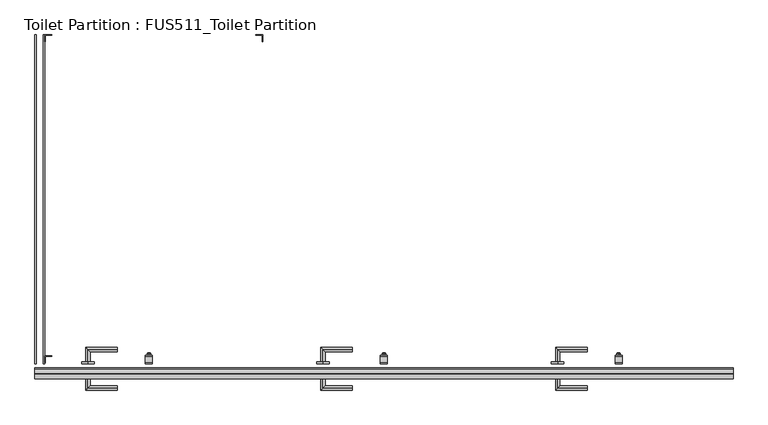
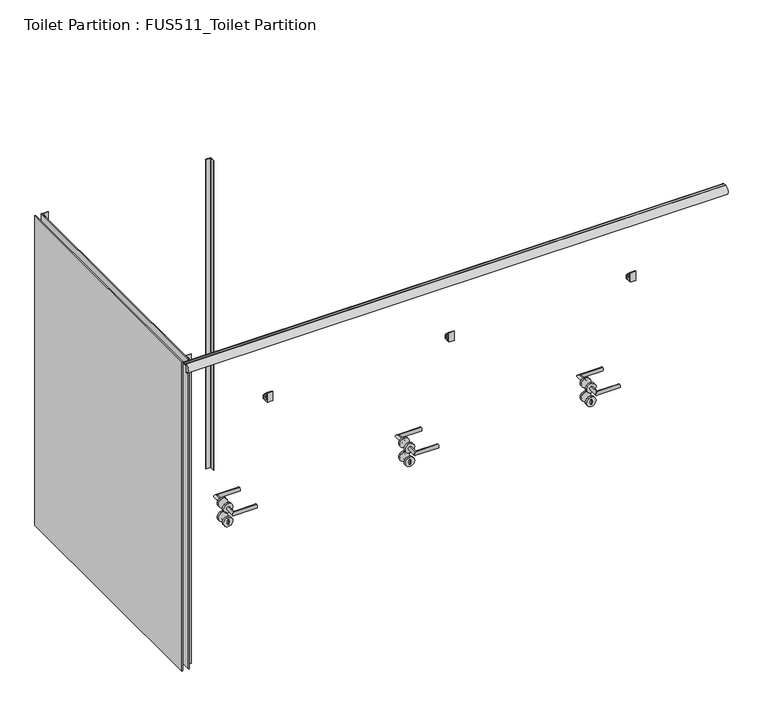
"""IFC4 building model written with IfcOpenShell, lengths in millimetres: furniture geometry, Toilet Partition : FUS511_Toilet Partition."""

from ifc_helpers import new_model, si_unit, point, frame, frame_2d, origin, place, context, project, spatial, polyline, circle_curve, ellipse_curve, trimmed, segment, composite_curve, outline, extrude, source, transform, mapped, element, save
from ifc_brep_helpers import plane_surface, cylinder_surface, revolved_surface, extruded_surface, advanced_brep


def toilet_partition_fus511_toilet_partition_80c0e7f6(model_context):
    return source(origin(), model_context, "Body", "SolidModel", [
        extrude(outline(composite_curve([segment(trimmed(circle_curve(frame_2d((-1451.3856706, 1892.2118377)), 1.0008364), [point((-1451.3856706, 1893.2126742))], [point((-1452.386507, 1892.2118377))], True, "CARTESIAN"), True, "CONTINUOUS"), segment(polyline([(-1452.386507, 1892.2118377), (-1452.386507, 1865.1892547), (-1453.3873434, 1865.1892547)]), True, "CONTINUOUS"), segment(trimmed(circle_curve(frame_2d((-1453.3873434, 1866.1900911)), 1.0008364), [point((-1453.3873434, 1865.1892547))], [point((-1454.3881798, 1866.1900911))], False, "CARTESIAN"), True, "CONTINUOUS"), segment(polyline([(-1454.3881798, 1866.1900911), (-1454.3881798, 1895.214347), (-1425.3639239, 1895.214347)]), True, "CONTINUOUS"), segment(trimmed(circle_curve(frame_2d((-1425.3639239, 1894.2135106)), 1.0008364), [point((-1425.3639239, 1895.214347))], [point((-1424.3630875, 1894.2135106))], False, "CARTESIAN"), True, "CONTINUOUS"), segment(polyline([(-1424.3630875, 1894.2135106), (-1424.3630875, 1893.2126742), (-1451.3856706, 1893.2126742)]), True, "CONTINUOUS")], self_intersect=False)), frame((0.0, 0.0, 100.0), z_axis=(0.0, 0.0, 1.0), x_axis=(1.0, 0.0, 0.0)), (0.0, 0.0, 1.0), 1800.0),
        extrude(outline(composite_curve([segment(trimmed(circle_curve(frame_2d((-1451.3856706, 527.0159753)), 1.0008364), [point((-1451.3856706, 528.0168117))], [point((-1452.386507, 527.0159753))], True, "CARTESIAN"), True, "CONTINUOUS"), segment(polyline([(-1452.386507, 527.0159753), (-1452.386507, 499.9933923), (-1453.3873434, 499.9933923)]), True, "CONTINUOUS"), segment(trimmed(circle_curve(frame_2d((-1453.3873434, 500.9942287)), 1.0008364), [point((-1453.3873434, 499.9933923))], [point((-1454.3881798, 500.9942287))], False, "CARTESIAN"), True, "CONTINUOUS"), segment(polyline([(-1454.3881798, 500.9942287), (-1454.3881798, 530.0184846), (-1425.3639239, 530.0184846)]), True, "CONTINUOUS"), segment(trimmed(circle_curve(frame_2d((-1425.3639239, 529.0176481)), 1.0008364), [point((-1425.3639239, 530.0184846))], [point((-1424.3630875, 529.0176481))], False, "CARTESIAN"), True, "CONTINUOUS"), segment(polyline([(-1424.3630875, 529.0176481), (-1424.3630875, 528.0168117), (-1451.3856706, 528.0168117)]), True, "CONTINUOUS")], self_intersect=False)), frame((0.0, 0.0, 100.0), z_axis=(0.0, 0.0, 1.0), x_axis=(1.0, 0.0, 0.0)), (0.0, 0.0, 1.0), 1800.0),
        extrude(outline(polyline([(-1454.3881798, 495.214347), (-1459.3881798, 495.214347), (-1459.3881798, 1895.214347), (-1454.3881798, 1895.214347), (-1454.3881798, 495.214347)])), frame((0.0, 0.0, 100.0), z_axis=(0.0, 0.0, 1.0), x_axis=(1.0, 0.0, 0.0)), (0.0, 0.0, 1.0), 1800.0),
        extrude(outline(polyline([(-1490.3881798, 495.214347), (-1495.3881798, 495.214347), (-1495.3881798, 1895.214347), (-1490.3881798, 1895.214347), (-1490.3881798, 495.214347)])), frame((0.0, 0.0, 100.0), z_axis=(0.0, 0.0, 1.0), x_axis=(1.0, 0.0, 0.0)), (0.0, 0.0, 1.0), 1800.0),
        advanced_brep(
        [(726.3556515, 505.214347, 893.5), (726.3556515, 505.214347, 946.5), (726.3556515, 505.214347, 934.6347495), (726.3556515, 505.214347, 904.6347495), (726.3556515, 495.214347, 893.5), (726.3556515, 495.214347, 946.5), (726.3556515, 499.9019579, 904.6347495), (726.3556515, 499.9019579, 934.6347495)],
        [
            (0, 1, circle_curve(frame((726.3556515, 505.214347, 920.0), z_axis=(0.0, 1.0, 0.0), x_axis=(0.0, 0.0, 1.0)), 26.5)),
            (1, 0, circle_curve(frame((726.3556515, 505.214347, 920.0), z_axis=(0.0, 1.0, 0.0), x_axis=(0.0, 0.0, 1.0)), 26.5)),
            (2, 3, ellipse_curve(frame((726.3556515, 505.214347, 919.6347495), z_axis=(0.0, -1.0, 0.0), x_axis=(0.0, 0.0, 1.0)), 15.0, 5.0)),
            (3, 2, ellipse_curve(frame((726.3556515, 505.214347, 919.6347495), z_axis=(0.0, -1.0, 0.0), x_axis=(0.0, 0.0, 1.0)), 15.0, 5.0)),
            (4, 5, circle_curve(frame((726.3556515, 495.214347, 920.0), z_axis=(0.0, -1.0, 0.0), x_axis=(0.0, 0.0, 1.0)), 26.5)),
            (5, 4, circle_curve(frame((726.3556515, 495.214347, 920.0), z_axis=(0.0, -1.0, 0.0), x_axis=(0.0, 0.0, 1.0)), 26.5)),
            (0, 4),
            (5, 1),
            (6, 7, ellipse_curve(frame((726.3556515, 499.9019579, 919.6347495), z_axis=(0.0, 1.0, 0.0), x_axis=(0.0, 0.0, 1.0)), 15.0, 5.0)),
            (7, 6, ellipse_curve(frame((726.3556515, 499.9019579, 919.6347495), z_axis=(0.0, 1.0, 0.0), x_axis=(0.0, 0.0, 1.0)), 15.0, 5.0)),
            (6, 3),
            (2, 7),
        ],
        [
            plane_surface(frame((726.3556515, 505.214347, 946.5), z_axis=(0.0, 1.0, 0.0), x_axis=(1.0, 0.0, 0.0))),
            plane_surface(frame((726.3556515, 495.214347, 946.5), z_axis=(0.0, -1.0, 0.0), x_axis=(-1.0, 0.0, 0.0))),
            cylinder_surface(frame((726.3556515, 495.214347, 920.0), z_axis=(0.0, 1.0, 0.0), x_axis=(0.0, 0.0, 1.0)), 26.5),
            plane_surface(frame((726.3556515, 499.9019579, 934.6347495), z_axis=(0.0, 1.0, 0.0), x_axis=(-1.0, 0.0, 0.0))),
            extruded_surface(trimmed(ellipse_curve(frame((726.3556515, 499.9019579, 919.6347495), z_axis=(0.0, 1.0, 0.0), x_axis=(0.0, 0.0, 1.0)), 15.0, 5.0), [point((726.3556515, 499.9019579, 904.6347495))], [point((726.3556515, 499.9019579, 934.6347495))], True, "CARTESIAN"), (0.0, -5.312388999999996, 0.0), 5.312388999999996),
            extruded_surface(trimmed(ellipse_curve(frame((726.3556515, 499.9019579, 919.6347495), z_axis=(0.0, 1.0, 0.0), x_axis=(0.0, 0.0, 1.0)), 15.0, 5.0), [point((726.3556515, 499.9019579, 934.6347495))], [point((726.3556515, 499.9019579, 904.6347495))], True, "CARTESIAN"), (0.0, -5.312388999999996, 0.0), 5.312388999999996),
        ],
        [
            (0, [[1, 2], [3, 4]]),
            (1, [[5, 6]]),
            (2, [[-1, 7, -6, 8]]),
            (2, [[-2, -8, -5, -7]]),
            (3, [[9, 10]]),
            (4, [[-9, 11, -3, 12]]),
            (5, [[-10, -12, -4, -11]]),
        ],
    ),
        advanced_brep(
        [(726.3556515, 505.214347, 990.5), (726.3556515, 505.214347, 1009.5), (726.3556515, 555.714347, 990.5), (726.3556515, 555.714347, 1009.5), (851.8556515, 555.714347, 990.5), (851.8556515, 555.714347, 1009.5)],
        [
            (0, 1, circle_curve(frame((726.3556515, 505.214347, 1000.0), z_axis=(0.0, -1.0, 0.0), x_axis=(0.0, 0.0, 1.0)), 9.5)),
            (1, 0, circle_curve(frame((726.3556515, 505.214347, 1000.0), z_axis=(0.0, -1.0, 0.0), x_axis=(0.0, 0.0, 1.0)), 9.5)),
            (0, 2),
            (2, 3, ellipse_curve(frame((726.3556515, 555.714347, 1000.0), z_axis=(-0.7071067811865486, -0.7071067811865465, 0.0), x_axis=(0.7071067811865465, -0.7071067811865485, 0.0)), 13.4350288, 9.5)),
            (3, 1),
            (3, 2, ellipse_curve(frame((726.3556515, 555.714347, 1000.0), z_axis=(-0.7071067811865486, -0.7071067811865465, 0.0), x_axis=(0.7071067811865465, -0.7071067811865485, 0.0)), 13.4350288, 9.5)),
            (4, 5, circle_curve(frame((851.8556515, 555.714347, 1000.0), z_axis=(1.0, 0.0, 0.0), x_axis=(0.0, 0.0, 1.0)), 9.5)),
            (5, 4, circle_curve(frame((851.8556515, 555.714347, 1000.0), z_axis=(1.0, 0.0, 0.0), x_axis=(0.0, 0.0, 1.0)), 9.5)),
            (2, 4),
            (5, 3),
        ],
        [
            plane_surface(frame((716.8556515, 505.214347, 1000.0), z_axis=(0.0, -1.0, 0.0), x_axis=(0.0, 0.0, 1.0))),
            cylinder_surface(frame((726.3556515, 505.214347, 1000.0), z_axis=(0.0, -1.0, 0.0), x_axis=(0.0, 0.0, 1.0)), 9.5),
            plane_surface(frame((851.8556515, 565.214347, 1000.0), z_axis=(1.0, 0.0, 0.0), x_axis=(0.0, 0.0, 1.0))),
            cylinder_surface(frame((716.8556515, 555.714347, 1000.0), z_axis=(-1.0, 0.0, 0.0), x_axis=(0.0, 0.0, 1.0)), 9.5),
        ],
        [
            (0, [[1, 2]]),
            (1, [[-1, 3, 4, 5]]),
            (1, [[-2, -5, 6, -3]]),
            (2, [[7, 8]]),
            (3, [[-4, 9, -8, 10]]),
            (3, [[-6, -10, -7, -9]]),
        ],
    ),
        extrude(outline(composite_curve([segment(trimmed(circle_curve(frame_2d((1000.0, 726.3556515)), 26.5), [point((973.5, 726.3556515))], [point((1026.5, 726.3556515))], False, "CARTESIAN"), True, "CONTINUOUS"), segment(trimmed(circle_curve(frame_2d((1000.0, 726.3556515)), 26.5), [point((1026.5, 726.3556515))], [point((973.5, 726.3556515))], False, "CARTESIAN"), True, "CONTINUOUS")], self_intersect=False)), frame((0.0, 495.214347, 0.0), z_axis=(0.0, 1.0, 0.0), x_axis=(0.0, 0.0, 1.0)), (0.0, 0.0, 1.0), 10.0),
        advanced_brep(
        [(-271.279512, 505.214347, 893.5), (-271.279512, 505.214347, 946.5), (-271.279512, 505.214347, 934.6347495), (-271.279512, 505.214347, 904.6347495), (-271.279512, 495.214347, 893.5), (-271.279512, 495.214347, 946.5), (-271.279512, 499.9019579, 904.6347495), (-271.279512, 499.9019579, 934.6347495)],
        [
            (0, 1, circle_curve(frame((-271.279512, 505.214347, 920.0), z_axis=(0.0, 1.0, 0.0), x_axis=(0.0, 0.0, 1.0)), 26.5)),
            (1, 0, circle_curve(frame((-271.279512, 505.214347, 920.0), z_axis=(0.0, 1.0, 0.0), x_axis=(0.0, 0.0, 1.0)), 26.5)),
            (2, 3, ellipse_curve(frame((-271.279512, 505.214347, 919.6347495), z_axis=(0.0, -1.0, 0.0), x_axis=(0.0, 0.0, 1.0)), 15.0, 5.0)),
            (3, 2, ellipse_curve(frame((-271.279512, 505.214347, 919.6347495), z_axis=(0.0, -1.0, 0.0), x_axis=(0.0, 0.0, 1.0)), 15.0, 5.0)),
            (4, 5, circle_curve(frame((-271.279512, 495.214347, 920.0), z_axis=(0.0, -1.0, 0.0), x_axis=(0.0, 0.0, 1.0)), 26.5)),
            (5, 4, circle_curve(frame((-271.279512, 495.214347, 920.0), z_axis=(0.0, -1.0, 0.0), x_axis=(0.0, 0.0, 1.0)), 26.5)),
            (0, 4),
            (5, 1),
            (6, 7, ellipse_curve(frame((-271.279512, 499.9019579, 919.6347495), z_axis=(0.0, 1.0, 0.0), x_axis=(0.0, 0.0, 1.0)), 15.0, 5.0)),
            (7, 6, ellipse_curve(frame((-271.279512, 499.9019579, 919.6347495), z_axis=(0.0, 1.0, 0.0), x_axis=(0.0, 0.0, 1.0)), 15.0, 5.0)),
            (6, 3),
            (2, 7),
        ],
        [
            plane_surface(frame((-271.279512, 505.214347, 946.5), z_axis=(0.0, 1.0, 0.0), x_axis=(1.0, 0.0, 0.0))),
            plane_surface(frame((-271.279512, 495.214347, 946.5), z_axis=(0.0, -1.0, 0.0), x_axis=(-1.0, 0.0, 0.0))),
            cylinder_surface(frame((-271.279512, 495.214347, 920.0), z_axis=(0.0, 1.0, 0.0), x_axis=(0.0, 0.0, 1.0)), 26.5),
            plane_surface(frame((-271.279512, 499.9019579, 934.6347495), z_axis=(0.0, 1.0, 0.0), x_axis=(-1.0, 0.0, 0.0))),
            extruded_surface(trimmed(ellipse_curve(frame((-271.279512, 499.9019579, 919.6347495), z_axis=(0.0, 1.0, 0.0), x_axis=(0.0, 0.0, 1.0)), 15.0, 5.0), [point((-271.279512, 499.9019579, 904.6347495))], [point((-271.279512, 499.9019579, 934.6347495))], True, "CARTESIAN"), (0.0, -5.312388999999996, 0.0), 5.312388999999996),
            extruded_surface(trimmed(ellipse_curve(frame((-271.279512, 499.9019579, 919.6347495), z_axis=(0.0, 1.0, 0.0), x_axis=(0.0, 0.0, 1.0)), 15.0, 5.0), [point((-271.279512, 499.9019579, 934.6347495))], [point((-271.279512, 499.9019579, 904.6347495))], True, "CARTESIAN"), (0.0, -5.312388999999996, 0.0), 5.312388999999996),
        ],
        [
            (0, [[1, 2], [3, 4]]),
            (1, [[5, 6]]),
            (2, [[-1, 7, -6, 8]]),
            (2, [[-2, -8, -5, -7]]),
            (3, [[9, 10]]),
            (4, [[-9, 11, -3, 12]]),
            (5, [[-10, -12, -4, -11]]),
        ],
    ),
        advanced_brep(
        [(-271.279512, 505.214347, 990.5), (-271.279512, 505.214347, 1009.5), (-271.279512, 555.714347, 990.5), (-271.279512, 555.714347, 1009.5), (-145.779512, 555.714347, 990.5), (-145.779512, 555.714347, 1009.5)],
        [
            (0, 1, circle_curve(frame((-271.279512, 505.214347, 1000.0), z_axis=(0.0, -1.0, 0.0), x_axis=(0.0, 0.0, 1.0)), 9.5)),
            (1, 0, circle_curve(frame((-271.279512, 505.214347, 1000.0), z_axis=(0.0, -1.0, 0.0), x_axis=(0.0, 0.0, 1.0)), 9.5)),
            (0, 2),
            (2, 3, ellipse_curve(frame((-271.279512, 555.714347, 1000.0), z_axis=(-0.7071067811865486, -0.7071067811865465, 0.0), x_axis=(0.7071067811865465, -0.7071067811865485, 0.0)), 13.4350288, 9.5)),
            (3, 1),
            (3, 2, ellipse_curve(frame((-271.279512, 555.714347, 1000.0), z_axis=(-0.7071067811865486, -0.7071067811865465, 0.0), x_axis=(0.7071067811865465, -0.7071067811865485, 0.0)), 13.4350288, 9.5)),
            (4, 5, circle_curve(frame((-145.779512, 555.714347, 1000.0), z_axis=(1.0, 0.0, 0.0), x_axis=(0.0, 0.0, 1.0)), 9.5)),
            (5, 4, circle_curve(frame((-145.779512, 555.714347, 1000.0), z_axis=(1.0, 0.0, 0.0), x_axis=(0.0, 0.0, 1.0)), 9.5)),
            (2, 4),
            (5, 3),
        ],
        [
            plane_surface(frame((-280.779512, 505.214347, 1000.0), z_axis=(0.0, -1.0, 0.0), x_axis=(0.0, 0.0, 1.0))),
            cylinder_surface(frame((-271.279512, 505.214347, 1000.0), z_axis=(0.0, -1.0, 0.0), x_axis=(0.0, 0.0, 1.0)), 9.5),
            plane_surface(frame((-145.779512, 565.214347, 1000.0), z_axis=(1.0, 0.0, 0.0), x_axis=(0.0, 0.0, 1.0))),
            cylinder_surface(frame((-280.779512, 555.714347, 1000.0), z_axis=(-1.0, 0.0, 0.0), x_axis=(0.0, 0.0, 1.0)), 9.5),
        ],
        [
            (0, [[1, 2]]),
            (1, [[-1, 3, 4, 5]]),
            (1, [[-2, -5, 6, -3]]),
            (2, [[7, 8]]),
            (3, [[-4, 9, -8, 10]]),
            (3, [[-6, -10, -7, -9]]),
        ],
    ),
        extrude(outline(composite_curve([segment(trimmed(circle_curve(frame_2d((1000.0, -271.279512)), 26.5), [point((973.5, -271.279512))], [point((1026.5, -271.279512))], False, "CARTESIAN"), True, "CONTINUOUS"), segment(trimmed(circle_curve(frame_2d((1000.0, -271.279512)), 26.5), [point((1026.5, -271.279512))], [point((973.5, -271.279512))], False, "CARTESIAN"), True, "CONTINUOUS")], self_intersect=False)), frame((0.0, 495.214347, 0.0), z_axis=(0.0, 1.0, 0.0), x_axis=(0.0, 0.0, 1.0)), (0.0, 0.0, 1.0), 10.0),
        advanced_brep(
        [(-1270.2108466, 505.214347, 893.5), (-1270.2108466, 505.214347, 946.5), (-1270.2108466, 505.214347, 934.6347495), (-1270.2108466, 505.214347, 904.6347495), (-1270.2108466, 495.214347, 893.5), (-1270.2108466, 495.214347, 946.5), (-1270.2108466, 499.9019579, 904.6347495), (-1270.2108466, 499.9019579, 934.6347495)],
        [
            (0, 1, circle_curve(frame((-1270.2108466, 505.214347, 920.0), z_axis=(0.0, 1.0, 0.0), x_axis=(0.0, 0.0, 1.0)), 26.5)),
            (1, 0, circle_curve(frame((-1270.2108466, 505.214347, 920.0), z_axis=(0.0, 1.0, 0.0), x_axis=(0.0, 0.0, 1.0)), 26.5)),
            (2, 3, ellipse_curve(frame((-1270.2108466, 505.214347, 919.6347495), z_axis=(0.0, -1.0, 0.0), x_axis=(0.0, 0.0, 1.0)), 15.0, 5.0)),
            (3, 2, ellipse_curve(frame((-1270.2108466, 505.214347, 919.6347495), z_axis=(0.0, -1.0, 0.0), x_axis=(0.0, 0.0, 1.0)), 15.0, 5.0)),
            (4, 5, circle_curve(frame((-1270.2108466, 495.214347, 920.0), z_axis=(0.0, -1.0, 0.0), x_axis=(0.0, 0.0, 1.0)), 26.5)),
            (5, 4, circle_curve(frame((-1270.2108466, 495.214347, 920.0), z_axis=(0.0, -1.0, 0.0), x_axis=(0.0, 0.0, 1.0)), 26.5)),
            (0, 4),
            (5, 1),
            (6, 7, ellipse_curve(frame((-1270.2108466, 499.9019579, 919.6347495), z_axis=(0.0, 1.0, 0.0), x_axis=(0.0, 0.0, 1.0)), 15.0, 5.0)),
            (7, 6, ellipse_curve(frame((-1270.2108466, 499.9019579, 919.6347495), z_axis=(0.0, 1.0, 0.0), x_axis=(0.0, 0.0, 1.0)), 15.0, 5.0)),
            (6, 3),
            (2, 7),
        ],
        [
            plane_surface(frame((-1270.2108466, 505.214347, 946.5), z_axis=(0.0, 1.0, 0.0), x_axis=(1.0, 0.0, 0.0))),
            plane_surface(frame((-1270.2108466, 495.214347, 946.5), z_axis=(0.0, -1.0, 0.0), x_axis=(-1.0, 0.0, 0.0))),
            cylinder_surface(frame((-1270.2108466, 495.214347, 920.0), z_axis=(0.0, 1.0, 0.0), x_axis=(0.0, 0.0, 1.0)), 26.5),
            plane_surface(frame((-1270.2108466, 499.9019579, 934.6347495), z_axis=(0.0, 1.0, 0.0), x_axis=(-1.0, 0.0, 0.0))),
            extruded_surface(trimmed(ellipse_curve(frame((-1270.2108466, 499.9019579, 919.6347495), z_axis=(0.0, 1.0, 0.0), x_axis=(0.0, 0.0, 1.0)), 15.0, 5.0), [point((-1270.2108466, 499.9019579, 904.6347495))], [point((-1270.2108466, 499.9019579, 934.6347495))], True, "CARTESIAN"), (0.0, -5.312388999999996, 0.0), 5.312388999999996),
            extruded_surface(trimmed(ellipse_curve(frame((-1270.2108466, 499.9019579, 919.6347495), z_axis=(0.0, 1.0, 0.0), x_axis=(0.0, 0.0, 1.0)), 15.0, 5.0), [point((-1270.2108466, 499.9019579, 934.6347495))], [point((-1270.2108466, 499.9019579, 904.6347495))], True, "CARTESIAN"), (0.0, -5.312388999999996, 0.0), 5.312388999999996),
        ],
        [
            (0, [[1, 2], [3, 4]]),
            (1, [[5, 6]]),
            (2, [[-1, 7, -6, 8]]),
            (2, [[-2, -8, -5, -7]]),
            (3, [[9, 10]]),
            (4, [[-9, 11, -3, 12]]),
            (5, [[-10, -12, -4, -11]]),
        ],
    ),
        advanced_brep(
        [(-1270.2108466, 505.214347, 990.5), (-1270.2108466, 505.214347, 1009.5), (-1270.2108466, 555.714347, 990.5), (-1270.2108466, 555.714347, 1009.5), (-1144.7108466, 555.714347, 990.5), (-1144.7108466, 555.714347, 1009.5)],
        [
            (0, 1, circle_curve(frame((-1270.2108466, 505.214347, 1000.0), z_axis=(0.0, -1.0, 0.0), x_axis=(0.0, 0.0, 1.0)), 9.5)),
            (1, 0, circle_curve(frame((-1270.2108466, 505.214347, 1000.0), z_axis=(0.0, -1.0, 0.0), x_axis=(0.0, 0.0, 1.0)), 9.5)),
            (0, 2),
            (2, 3, ellipse_curve(frame((-1270.2108466, 555.714347, 1000.0), z_axis=(-0.7071067811865486, -0.7071067811865465, 0.0), x_axis=(0.7071067811865465, -0.7071067811865485, 0.0)), 13.4350288, 9.5)),
            (3, 1),
            (3, 2, ellipse_curve(frame((-1270.2108466, 555.714347, 1000.0), z_axis=(-0.7071067811865486, -0.7071067811865465, 0.0), x_axis=(0.7071067811865465, -0.7071067811865485, 0.0)), 13.4350288, 9.5)),
            (4, 5, circle_curve(frame((-1144.7108466, 555.714347, 1000.0), z_axis=(1.0, 0.0, 0.0), x_axis=(0.0, 0.0, 1.0)), 9.5)),
            (5, 4, circle_curve(frame((-1144.7108466, 555.714347, 1000.0), z_axis=(1.0, 0.0, 0.0), x_axis=(0.0, 0.0, 1.0)), 9.5)),
            (2, 4),
            (5, 3),
        ],
        [
            plane_surface(frame((-1279.7108466, 505.214347, 1000.0), z_axis=(0.0, -1.0, 0.0), x_axis=(0.0, 0.0, 1.0))),
            cylinder_surface(frame((-1270.2108466, 505.214347, 1000.0), z_axis=(0.0, -1.0, 0.0), x_axis=(0.0, 0.0, 1.0)), 9.5),
            plane_surface(frame((-1144.7108466, 565.214347, 1000.0), z_axis=(1.0, 0.0, 0.0), x_axis=(0.0, 0.0, 1.0))),
            cylinder_surface(frame((-1279.7108466, 555.714347, 1000.0), z_axis=(-1.0, 0.0, 0.0), x_axis=(0.0, 0.0, 1.0)), 9.5),
        ],
        [
            (0, [[1, 2]]),
            (1, [[-1, 3, 4, 5]]),
            (1, [[-2, -5, 6, -3]]),
            (2, [[7, 8]]),
            (3, [[-4, 9, -8, 10]]),
            (3, [[-6, -10, -7, -9]]),
        ],
    ),
        extrude(outline(composite_curve([segment(trimmed(circle_curve(frame_2d((1000.0, -1270.2108466)), 26.5), [point((973.5, -1270.2108466))], [point((1026.5, -1270.2108466))], False, "CARTESIAN"), True, "CONTINUOUS"), segment(trimmed(circle_curve(frame_2d((1000.0, -1270.2108466)), 26.5), [point((1026.5, -1270.2108466))], [point((973.5, -1270.2108466))], False, "CARTESIAN"), True, "CONTINUOUS")], self_intersect=False)), frame((0.0, 495.214347, 0.0), z_axis=(0.0, 1.0, 0.0), x_axis=(0.0, 0.0, 1.0)), (0.0, 0.0, 1.0), 10.0),
        advanced_brep(
        [(726.3556515, 444.214347, 893.5), (726.3556515, 444.214347, 946.5), (726.3556515, 444.214347, 934.6347495), (726.3556515, 444.214347, 904.6347495), (726.3556515, 454.214347, 893.5), (726.3556515, 454.214347, 946.5), (726.3556515, 449.526736, 904.6347495), (726.3556515, 449.526736, 934.6347495)],
        [
            (0, 1, circle_curve(frame((726.3556515, 444.214347, 920.0), z_axis=(0.0, -1.0, 0.0), x_axis=(0.0, 0.0, 1.0)), 26.5)),
            (1, 0, circle_curve(frame((726.3556515, 444.214347, 920.0), z_axis=(0.0, -1.0, 0.0), x_axis=(0.0, 0.0, 1.0)), 26.5)),
            (2, 3, ellipse_curve(frame((726.3556515, 444.214347, 919.6347495), z_axis=(0.0, 1.0, 0.0), x_axis=(0.0, 0.0, 1.0)), 15.0, 5.0)),
            (3, 2, ellipse_curve(frame((726.3556515, 444.214347, 919.6347495), z_axis=(0.0, 1.0, 0.0), x_axis=(0.0, 0.0, 1.0)), 15.0, 5.0)),
            (4, 5, circle_curve(frame((726.3556515, 454.214347, 920.0), z_axis=(0.0, 1.0, 0.0), x_axis=(0.0, 0.0, 1.0)), 26.5)),
            (5, 4, circle_curve(frame((726.3556515, 454.214347, 920.0), z_axis=(0.0, 1.0, 0.0), x_axis=(0.0, 0.0, 1.0)), 26.5)),
            (1, 5),
            (4, 0),
            (6, 7, ellipse_curve(frame((726.3556515, 449.526736, 919.6347495), z_axis=(0.0, -1.0, 0.0), x_axis=(0.0, 0.0, 1.0)), 15.0, 5.0)),
            (7, 6, ellipse_curve(frame((726.3556515, 449.526736, 919.6347495), z_axis=(0.0, -1.0, 0.0), x_axis=(0.0, 0.0, 1.0)), 15.0, 5.0)),
            (7, 2),
            (3, 6),
        ],
        [
            plane_surface(frame((726.3556515, 444.214347, 946.5), z_axis=(0.0, -1.0, 0.0), x_axis=(1.0, 0.0, 0.0))),
            plane_surface(frame((726.3556515, 454.214347, 946.5), z_axis=(0.0, 1.0, 0.0), x_axis=(-1.0, 0.0, 0.0))),
            cylinder_surface(frame((726.3556515, 454.214347, 920.0), z_axis=(0.0, -1.0, 0.0), x_axis=(0.0, 0.0, 1.0)), 26.5),
            plane_surface(frame((726.3556515, 449.526736, 934.6347495), z_axis=(0.0, -1.0, 0.0), x_axis=(-1.0, 0.0, 0.0))),
            extruded_surface(trimmed(ellipse_curve(frame((726.3556515, 454.8391251, 919.6347495), z_axis=(0.0, 1.0, 0.0), x_axis=(0.0, 0.0, 1.0)), 15.0, 5.0), [point((726.3556515, 454.8391251, 904.6347495))], [point((726.3556515, 454.8391251, 934.6347495))], True, "CARTESIAN"), (0.0, -5.312389099999962, 0.0), 5.312389099999962),
            extruded_surface(trimmed(ellipse_curve(frame((726.3556515, 454.8391251, 919.6347495), z_axis=(0.0, 1.0, 0.0), x_axis=(0.0, 0.0, 1.0)), 15.0, 5.0), [point((726.3556515, 454.8391251, 934.6347495))], [point((726.3556515, 454.8391251, 904.6347495))], True, "CARTESIAN"), (0.0, -5.312389099999962, 0.0), 5.312389099999962),
        ],
        [
            (0, [[1, 2], [3, 4]]),
            (1, [[5, 6]]),
            (2, [[7, -5, 8, -2]]),
            (2, [[-8, -6, -7, -1]]),
            (3, [[9, 10]]),
            (4, [[11, -4, 12, -10]]),
            (5, [[-12, -3, -11, -9]]),
        ],
    ),
        advanced_brep(
        [(726.3556515, 444.214347, 990.5), (726.3556515, 444.214347, 1009.5), (726.3556515, 393.714347, 1009.5), (726.3556515, 393.714347, 990.5), (851.8556515, 393.714347, 990.5), (851.8556515, 393.714347, 1009.5)],
        [
            (0, 1, circle_curve(frame((726.3556515, 444.214347, 1000.0), z_axis=(0.0, 1.0, 0.0), x_axis=(0.0, 0.0, 1.0)), 9.5)),
            (1, 0, circle_curve(frame((726.3556515, 444.214347, 1000.0), z_axis=(0.0, 1.0, 0.0), x_axis=(0.0, 0.0, 1.0)), 9.5)),
            (1, 2),
            (2, 3, ellipse_curve(frame((726.3556515, 393.714347, 1000.0), z_axis=(-0.7071067811865486, 0.7071067811865465, 0.0), x_axis=(0.7071067811865465, 0.7071067811865485, 0.0)), 13.4350288, 9.5)),
            (3, 0),
            (3, 2, ellipse_curve(frame((726.3556515, 393.714347, 1000.0), z_axis=(-0.7071067811865486, 0.7071067811865465, 0.0), x_axis=(0.7071067811865465, 0.7071067811865485, 0.0)), 13.4350288, 9.5)),
            (4, 5, circle_curve(frame((851.8556515, 393.714347, 1000.0), z_axis=(1.0, 0.0, 0.0), x_axis=(0.0, 0.0, 1.0)), 9.5)),
            (5, 4, circle_curve(frame((851.8556515, 393.714347, 1000.0), z_axis=(1.0, 0.0, 0.0), x_axis=(0.0, 0.0, 1.0)), 9.5)),
            (2, 5),
            (4, 3),
        ],
        [
            plane_surface(frame((716.8556515, 444.214347, 1000.0), z_axis=(0.0, 1.0, 0.0), x_axis=(0.0, 0.0, 1.0))),
            cylinder_surface(frame((726.3556515, 444.214347, 1000.0), z_axis=(0.0, 1.0, 0.0), x_axis=(0.0, 0.0, 1.0)), 9.5),
            plane_surface(frame((851.8556515, 384.214347, 1000.0), z_axis=(1.0, 0.0, 0.0), x_axis=(0.0, 0.0, 1.0))),
            cylinder_surface(frame((716.8556515, 393.714347, 1000.0), z_axis=(-1.0, 0.0, 0.0), x_axis=(0.0, 0.0, 1.0)), 9.5),
        ],
        [
            (0, [[1, 2]]),
            (1, [[3, 4, 5, -2]]),
            (1, [[-5, 6, -3, -1]]),
            (2, [[7, 8]]),
            (3, [[9, -7, 10, -4]]),
            (3, [[-10, -8, -9, -6]]),
        ],
    ),
        extrude(outline(composite_curve([segment(trimmed(circle_curve(frame_2d((1000.0, 726.3556515)), 26.5), [point((973.5, 726.3556515))], [point((1026.5, 726.3556515))], False, "CARTESIAN"), True, "CONTINUOUS"), segment(trimmed(circle_curve(frame_2d((1000.0, 726.3556515)), 26.5), [point((1026.5, 726.3556515))], [point((973.5, 726.3556515))], False, "CARTESIAN"), True, "CONTINUOUS")], self_intersect=False)), frame((0.0, 444.214347, 0.0), z_axis=(0.0, 1.0, 0.0), x_axis=(0.0, 0.0, 1.0)), (0.0, 0.0, 1.0), 10.0),
        advanced_brep(
        [(-271.279512, 444.214347, 893.5), (-271.279512, 444.214347, 946.5), (-271.279512, 444.214347, 934.6347495), (-271.279512, 444.214347, 904.6347495), (-271.279512, 454.214347, 893.5), (-271.279512, 454.214347, 946.5), (-271.279512, 449.526736, 904.6347495), (-271.279512, 449.526736, 934.6347495)],
        [
            (0, 1, circle_curve(frame((-271.279512, 444.214347, 920.0), z_axis=(0.0, -1.0, 0.0), x_axis=(0.0, 0.0, 1.0)), 26.5)),
            (1, 0, circle_curve(frame((-271.279512, 444.214347, 920.0), z_axis=(0.0, -1.0, 0.0), x_axis=(0.0, 0.0, 1.0)), 26.5)),
            (2, 3, ellipse_curve(frame((-271.279512, 444.214347, 919.6347495), z_axis=(0.0, 1.0, 0.0), x_axis=(0.0, 0.0, 1.0)), 15.0, 5.0)),
            (3, 2, ellipse_curve(frame((-271.279512, 444.214347, 919.6347495), z_axis=(0.0, 1.0, 0.0), x_axis=(0.0, 0.0, 1.0)), 15.0, 5.0)),
            (4, 5, circle_curve(frame((-271.279512, 454.214347, 920.0), z_axis=(0.0, 1.0, 0.0), x_axis=(0.0, 0.0, 1.0)), 26.5)),
            (5, 4, circle_curve(frame((-271.279512, 454.214347, 920.0), z_axis=(0.0, 1.0, 0.0), x_axis=(0.0, 0.0, 1.0)), 26.5)),
            (1, 5),
            (4, 0),
            (6, 7, ellipse_curve(frame((-271.279512, 449.526736, 919.6347495), z_axis=(0.0, -1.0, 0.0), x_axis=(0.0, 0.0, 1.0)), 15.0, 5.0)),
            (7, 6, ellipse_curve(frame((-271.279512, 449.526736, 919.6347495), z_axis=(0.0, -1.0, 0.0), x_axis=(0.0, 0.0, 1.0)), 15.0, 5.0)),
            (7, 2),
            (3, 6),
        ],
        [
            plane_surface(frame((-271.279512, 444.214347, 946.5), z_axis=(0.0, -1.0, 0.0), x_axis=(1.0, 0.0, 0.0))),
            plane_surface(frame((-271.279512, 454.214347, 946.5), z_axis=(0.0, 1.0, 0.0), x_axis=(-1.0, 0.0, 0.0))),
            cylinder_surface(frame((-271.279512, 454.214347, 920.0), z_axis=(0.0, -1.0, 0.0), x_axis=(0.0, 0.0, 1.0)), 26.5),
            plane_surface(frame((-271.279512, 449.526736, 934.6347495), z_axis=(0.0, -1.0, 0.0), x_axis=(-1.0, 0.0, 0.0))),
            extruded_surface(trimmed(ellipse_curve(frame((-271.279512, 454.8391251, 919.6347495), z_axis=(0.0, 1.0, 0.0), x_axis=(0.0, 0.0, 1.0)), 15.0, 5.0), [point((-271.279512, 454.8391251, 904.6347495))], [point((-271.279512, 454.8391251, 934.6347495))], True, "CARTESIAN"), (0.0, -5.312389099999962, 0.0), 5.312389099999962),
            extruded_surface(trimmed(ellipse_curve(frame((-271.279512, 454.8391251, 919.6347495), z_axis=(0.0, 1.0, 0.0), x_axis=(0.0, 0.0, 1.0)), 15.0, 5.0), [point((-271.279512, 454.8391251, 934.6347495))], [point((-271.279512, 454.8391251, 904.6347495))], True, "CARTESIAN"), (0.0, -5.312389099999962, 0.0), 5.312389099999962),
        ],
        [
            (0, [[1, 2], [3, 4]]),
            (1, [[5, 6]]),
            (2, [[7, -5, 8, -2]]),
            (2, [[-8, -6, -7, -1]]),
            (3, [[9, 10]]),
            (4, [[11, -4, 12, -10]]),
            (5, [[-12, -3, -11, -9]]),
        ],
    ),
        advanced_brep(
        [(-271.279512, 444.214347, 990.5), (-271.279512, 444.214347, 1009.5), (-271.279512, 393.714347, 1009.5), (-271.279512, 393.714347, 990.5), (-145.779512, 393.714347, 990.5), (-145.779512, 393.714347, 1009.5)],
        [
            (0, 1, circle_curve(frame((-271.279512, 444.214347, 1000.0), z_axis=(0.0, 1.0, 0.0), x_axis=(0.0, 0.0, 1.0)), 9.5)),
            (1, 0, circle_curve(frame((-271.279512, 444.214347, 1000.0), z_axis=(0.0, 1.0, 0.0), x_axis=(0.0, 0.0, 1.0)), 9.5)),
            (1, 2),
            (2, 3, ellipse_curve(frame((-271.279512, 393.714347, 1000.0), z_axis=(-0.7071067811865486, 0.7071067811865465, 0.0), x_axis=(0.7071067811865465, 0.7071067811865485, 0.0)), 13.4350288, 9.5)),
            (3, 0),
            (3, 2, ellipse_curve(frame((-271.279512, 393.714347, 1000.0), z_axis=(-0.7071067811865486, 0.7071067811865465, 0.0), x_axis=(0.7071067811865465, 0.7071067811865485, 0.0)), 13.4350288, 9.5)),
            (4, 5, circle_curve(frame((-145.779512, 393.714347, 1000.0), z_axis=(1.0, 0.0, 0.0), x_axis=(0.0, 0.0, 1.0)), 9.5)),
            (5, 4, circle_curve(frame((-145.779512, 393.714347, 1000.0), z_axis=(1.0, 0.0, 0.0), x_axis=(0.0, 0.0, 1.0)), 9.5)),
            (2, 5),
            (4, 3),
        ],
        [
            plane_surface(frame((-280.779512, 444.214347, 1000.0), z_axis=(0.0, 1.0, 0.0), x_axis=(0.0, 0.0, 1.0))),
            cylinder_surface(frame((-271.279512, 444.214347, 1000.0), z_axis=(0.0, 1.0, 0.0), x_axis=(0.0, 0.0, 1.0)), 9.5),
            plane_surface(frame((-145.779512, 384.214347, 1000.0), z_axis=(1.0, 0.0, 0.0), x_axis=(0.0, 0.0, 1.0))),
            cylinder_surface(frame((-280.779512, 393.714347, 1000.0), z_axis=(-1.0, 0.0, 0.0), x_axis=(0.0, 0.0, 1.0)), 9.5),
        ],
        [
            (0, [[1, 2]]),
            (1, [[3, 4, 5, -2]]),
            (1, [[-5, 6, -3, -1]]),
            (2, [[7, 8]]),
            (3, [[9, -7, 10, -4]]),
            (3, [[-10, -8, -9, -6]]),
        ],
    ),
        extrude(outline(composite_curve([segment(trimmed(circle_curve(frame_2d((1000.0, -271.279512)), 26.5), [point((973.5, -271.279512))], [point((1026.5, -271.279512))], False, "CARTESIAN"), True, "CONTINUOUS"), segment(trimmed(circle_curve(frame_2d((1000.0, -271.279512)), 26.5), [point((1026.5, -271.279512))], [point((973.5, -271.279512))], False, "CARTESIAN"), True, "CONTINUOUS")], self_intersect=False)), frame((0.0, 444.214347, 0.0), z_axis=(0.0, 1.0, 0.0), x_axis=(0.0, 0.0, 1.0)), (0.0, 0.0, 1.0), 10.0),
        advanced_brep(
        [(-1270.2108466, 444.214347, 893.5), (-1270.2108466, 444.214347, 946.5), (-1270.2108466, 444.214347, 934.6347495), (-1270.2108466, 444.214347, 904.6347495), (-1270.2108466, 454.214347, 893.5), (-1270.2108466, 454.214347, 946.5), (-1270.2108466, 449.526736, 904.6347495), (-1270.2108466, 449.526736, 934.6347495)],
        [
            (0, 1, circle_curve(frame((-1270.2108466, 444.214347, 920.0), z_axis=(0.0, -1.0, 0.0), x_axis=(0.0, 0.0, 1.0)), 26.5)),
            (1, 0, circle_curve(frame((-1270.2108466, 444.214347, 920.0), z_axis=(0.0, -1.0, 0.0), x_axis=(0.0, 0.0, 1.0)), 26.5)),
            (2, 3, ellipse_curve(frame((-1270.2108466, 444.214347, 919.6347495), z_axis=(0.0, 1.0, 0.0), x_axis=(0.0, 0.0, 1.0)), 15.0, 5.0)),
            (3, 2, ellipse_curve(frame((-1270.2108466, 444.214347, 919.6347495), z_axis=(0.0, 1.0, 0.0), x_axis=(0.0, 0.0, 1.0)), 15.0, 5.0)),
            (4, 5, circle_curve(frame((-1270.2108466, 454.214347, 920.0), z_axis=(0.0, 1.0, 0.0), x_axis=(0.0, 0.0, 1.0)), 26.5)),
            (5, 4, circle_curve(frame((-1270.2108466, 454.214347, 920.0), z_axis=(0.0, 1.0, 0.0), x_axis=(0.0, 0.0, 1.0)), 26.5)),
            (1, 5),
            (4, 0),
            (6, 7, ellipse_curve(frame((-1270.2108466, 449.526736, 919.6347495), z_axis=(0.0, -1.0, 0.0), x_axis=(0.0, 0.0, 1.0)), 15.0, 5.0)),
            (7, 6, ellipse_curve(frame((-1270.2108466, 449.526736, 919.6347495), z_axis=(0.0, -1.0, 0.0), x_axis=(0.0, 0.0, 1.0)), 15.0, 5.0)),
            (7, 2),
            (3, 6),
        ],
        [
            plane_surface(frame((-1270.2108466, 444.214347, 946.5), z_axis=(0.0, -1.0, 0.0), x_axis=(1.0, 0.0, 0.0))),
            plane_surface(frame((-1270.2108466, 454.214347, 946.5), z_axis=(0.0, 1.0, 0.0), x_axis=(-1.0, 0.0, 0.0))),
            cylinder_surface(frame((-1270.2108466, 454.214347, 920.0), z_axis=(0.0, -1.0, 0.0), x_axis=(0.0, 0.0, 1.0)), 26.5),
            plane_surface(frame((-1270.2108466, 449.526736, 934.6347495), z_axis=(0.0, -1.0, 0.0), x_axis=(-1.0, 0.0, 0.0))),
            extruded_surface(trimmed(ellipse_curve(frame((-1270.2108466, 454.8391251, 919.6347495), z_axis=(0.0, 1.0, 0.0), x_axis=(0.0, 0.0, 1.0)), 15.0, 5.0), [point((-1270.2108466, 454.8391251, 904.6347495))], [point((-1270.2108466, 454.8391251, 934.6347495))], True, "CARTESIAN"), (0.0, -5.312389099999962, 0.0), 5.312389099999962),
            extruded_surface(trimmed(ellipse_curve(frame((-1270.2108466, 454.8391251, 919.6347495), z_axis=(0.0, 1.0, 0.0), x_axis=(0.0, 0.0, 1.0)), 15.0, 5.0), [point((-1270.2108466, 454.8391251, 934.6347495))], [point((-1270.2108466, 454.8391251, 904.6347495))], True, "CARTESIAN"), (0.0, -5.312389099999962, 0.0), 5.312389099999962),
        ],
        [
            (0, [[1, 2], [3, 4]]),
            (1, [[5, 6]]),
            (2, [[7, -5, 8, -2]]),
            (2, [[-8, -6, -7, -1]]),
            (3, [[9, 10]]),
            (4, [[11, -4, 12, -10]]),
            (5, [[-12, -3, -11, -9]]),
        ],
    ),
        advanced_brep(
        [(-1270.2108466, 444.214347, 990.5), (-1270.2108466, 444.214347, 1009.5), (-1270.2108466, 393.714347, 1009.5), (-1270.2108466, 393.714347, 990.5), (-1144.7108466, 393.714347, 990.5), (-1144.7108466, 393.714347, 1009.5)],
        [
            (0, 1, circle_curve(frame((-1270.2108466, 444.214347, 1000.0), z_axis=(0.0, 1.0, 0.0), x_axis=(0.0, 0.0, 1.0)), 9.5)),
            (1, 0, circle_curve(frame((-1270.2108466, 444.214347, 1000.0), z_axis=(0.0, 1.0, 0.0), x_axis=(0.0, 0.0, 1.0)), 9.5)),
            (1, 2),
            (2, 3, ellipse_curve(frame((-1270.2108466, 393.714347, 1000.0), z_axis=(-0.7071067811865486, 0.7071067811865465, 0.0), x_axis=(0.7071067811865465, 0.7071067811865485, 0.0)), 13.4350288, 9.5)),
            (3, 0),
            (3, 2, ellipse_curve(frame((-1270.2108466, 393.714347, 1000.0), z_axis=(-0.7071067811865486, 0.7071067811865465, 0.0), x_axis=(0.7071067811865465, 0.7071067811865485, 0.0)), 13.4350288, 9.5)),
            (4, 5, circle_curve(frame((-1144.7108466, 393.714347, 1000.0), z_axis=(1.0, 0.0, 0.0), x_axis=(0.0, 0.0, 1.0)), 9.5)),
            (5, 4, circle_curve(frame((-1144.7108466, 393.714347, 1000.0), z_axis=(1.0, 0.0, 0.0), x_axis=(0.0, 0.0, 1.0)), 9.5)),
            (2, 5),
            (4, 3),
        ],
        [
            plane_surface(frame((-1279.7108466, 444.214347, 1000.0), z_axis=(0.0, 1.0, 0.0), x_axis=(0.0, 0.0, 1.0))),
            cylinder_surface(frame((-1270.2108466, 444.214347, 1000.0), z_axis=(0.0, 1.0, 0.0), x_axis=(0.0, 0.0, 1.0)), 9.5),
            plane_surface(frame((-1144.7108466, 384.214347, 1000.0), z_axis=(1.0, 0.0, 0.0), x_axis=(0.0, 0.0, 1.0))),
            cylinder_surface(frame((-1279.7108466, 393.714347, 1000.0), z_axis=(-1.0, 0.0, 0.0), x_axis=(0.0, 0.0, 1.0)), 9.5),
        ],
        [
            (0, [[1, 2]]),
            (1, [[3, 4, 5, -2]]),
            (1, [[-5, 6, -3, -1]]),
            (2, [[7, 8]]),
            (3, [[9, -7, 10, -4]]),
            (3, [[-10, -8, -9, -6]]),
        ],
    ),
        extrude(outline(composite_curve([segment(trimmed(circle_curve(frame_2d((1000.0, -1270.2108466)), 26.5), [point((973.5, -1270.2108466))], [point((1026.5, -1270.2108466))], False, "CARTESIAN"), True, "CONTINUOUS"), segment(trimmed(circle_curve(frame_2d((1000.0, -1270.2108466)), 26.5), [point((1026.5, -1270.2108466))], [point((973.5, -1270.2108466))], False, "CARTESIAN"), True, "CONTINUOUS")], self_intersect=False)), frame((0.0, 444.214347, 0.0), z_axis=(0.0, 1.0, 0.0), x_axis=(0.0, 0.0, 1.0)), (0.0, 0.0, 1.0), 10.0),
        extrude(outline(composite_curve([segment(trimmed(circle_curve(frame_2d((458.4868618, 1888.0268612)), 26.5042707), [point((454.214347, 1861.869224))], [point((453.0212869, 1913.9614685))], False, "CARTESIAN"), True, "CONTINUOUS"), segment(trimmed(circle_curve(frame_2d((453.1556919, 1912.91138)), 1.058655), [point((453.0212869, 1913.9614685))], [point((454.214347, 1912.91138))], False, "CARTESIAN"), True, "CONTINUOUS"), segment(polyline([(454.214347, 1912.91138), (454.214347, 1909.5278954), (474.6592543, 1909.5278954)]), True, "CONTINUOUS"), segment(trimmed(circle_curve(frame_2d((474.2293597, 1904.6828737)), 4.8640564), [point((474.6592543, 1909.5278954))], [point((479.0927404, 1904.7639477))], False, "CARTESIAN"), True, "CONTINUOUS"), segment(trimmed(circle_curve(frame_2d((474.2293597, 1904.8450217)), 4.8640564), [point((479.0927404, 1904.7639477))], [point((473.7994652, 1900.0))], False, "CARTESIAN"), True, "CONTINUOUS"), segment(polyline([(473.7994652, 1900.0), (454.214347, 1900.0), (454.214347, 1861.869224)]), True, "CONTINUOUS")], self_intersect=False), holes=[composite_curve([segment(polyline([(473.939812, 1907.9461271), (455.8017383, 1907.9399126), (455.8017383, 1901.5879827), (473.9398142, 1901.5817682)]), True, "CONTINUOUS"), segment(trimmed(circle_curve(frame_2d((473.9325063, 1904.7639477)), 3.1821878), [point((473.9398142, 1901.5817682))], [point((473.939812, 1907.9461271))], True, "CARTESIAN"), True, "CONTINUOUS")], self_intersect=False), composite_curve([segment(trimmed(circle_curve(frame_2d((457.6658618, 1888.0268612)), 24.6245189), [point((452.6263644, 1912.1301887))], [point((452.6263644, 1863.9235337))], True, "CARTESIAN"), True, "CONTINUOUS"), segment(polyline([(452.6263644, 1863.9235337), (452.6263644, 1912.1301887)]), True, "CONTINUOUS")], self_intersect=False)]), frame((-1495.4101478, 0.0, 0.0), z_axis=(1.0, 0.0, 0.0), x_axis=(0.0, 1.0, 0.0)), (0.0, 0.0, 1.0), 2967.0),
        extrude(outline(composite_curve([segment(polyline([(499.2367016, 1553.2961991), (499.2367016, 1504.0), (527.3931841, 1504.0), (527.3931841, 1516.0894186)]), True, "CONTINUOUS"), segment(trimmed(circle_curve(frame_2d((531.4155388, 1516.0894186)), 4.0223546), [point((527.3931841, 1516.0894186))], [point((531.4155388, 1520.1117732))], False, "CARTESIAN"), True, "CONTINUOUS"), segment(polyline([(531.4155388, 1520.1117732), (531.4155388, 1500.0), (499.2367016, 1500.0), (495.214347, 1500.0), (495.214347, 1553.2961991), (499.2367016, 1553.2961991)]), True, "CONTINUOUS")], self_intersect=False)), frame((-1026.1694992, 0.0, 0.0), z_axis=(1.0, 0.0, 0.0), x_axis=(0.0, 1.0, 0.0)), (0.0, 0.0, 1.0), 30.0),
        advanced_brep(
        [(-1011.1694992, 531.4155388, 1510.5586809), (-1011.1694992, 531.4155388, 1518.1005959), (-1011.1694992, 531.4155388, 1503.016766), (-1011.1694992, 541.4714254, 1506.033532), (-1011.1694992, 541.4714254, 1515.0838299), (-1011.1694992, 541.4714254, 1510.5586809), (-1011.1694992, 539.4602481, 1503.016766), (-1011.1694992, 539.4602481, 1518.1005959)],
        [
            (0, 1),
            (1, 2, circle_curve(frame((-1011.1694992, 531.4155388, 1510.5586809), z_axis=(0.0, -1.0, 0.0), x_axis=(0.0, 0.0, 1.0)), 7.541915)),
            (2, 0),
            (2, 1, circle_curve(frame((-1011.1694992, 531.4155388, 1510.5586809), z_axis=(0.0, -1.0, 0.0), x_axis=(0.0, 0.0, 1.0)), 7.541915)),
            (3, 4, circle_curve(frame((-1011.1694992, 541.4714254, 1510.5586809), z_axis=(0.0, 1.0, 0.0), x_axis=(0.0, 0.0, 1.0)), 4.525149)),
            (4, 5),
            (5, 3),
            (4, 3, circle_curve(frame((-1011.1694992, 541.4714254, 1510.5586809), z_axis=(0.0, 1.0, 0.0), x_axis=(0.0, 0.0, 1.0)), 4.525149)),
            (6, 7, circle_curve(frame((-1011.1694992, 539.4602481, 1510.5586809), z_axis=(0.0, 1.0, 0.0), x_axis=(0.0, 0.0, 1.0)), 7.541915)),
            (7, 4, circle_curve(frame((-1011.1694992, 538.111954, 1515.0229578), z_axis=(-1.0, 0.0, 0.0), x_axis=(0.0, 0.0, -1.0)), 3.3600228)),
            (3, 6, circle_curve(frame((-1011.1694992, 538.111954, 1506.0944041), z_axis=(-1.0, 0.0, 0.0), x_axis=(0.0, 0.0, 1.0)), 3.3600228)),
            (7, 6, circle_curve(frame((-1011.1694992, 539.4602481, 1510.5586809), z_axis=(0.0, 1.0, 0.0), x_axis=(0.0, 0.0, 1.0)), 7.541915)),
            (1, 7),
            (6, 2),
        ],
        [
            plane_surface(frame((-1011.1694992, 531.4155388, 1510.5586809), z_axis=(0.0, -1.0, 0.0), x_axis=(0.0, 0.0, 1.0))),
            plane_surface(frame((-1011.1694992, 541.4714254, 1510.5586809), z_axis=(0.0, 1.0, 0.0), x_axis=(0.0, 0.0, 1.0))),
            revolved_surface(trimmed(ellipse_curve(frame((-1011.1694992, 538.111954, 1515.0229578), z_axis=(1.0, 0.0, 0.0), x_axis=(0.0, 0.0, -1.0)), 3.3600228, 3.3600228), [point((-1011.1694992, 541.4714254, 1515.0838299))], [point((-1011.1694992, 539.4602481, 1518.1005959))], True, "CARTESIAN"), (-1011.1694992, 521.4714254, 1510.5586809), (0.0, -1.0, 0.0)),
            cylinder_surface(frame((-1011.1694992, 521.4714254, 1510.5586809), z_axis=(0.0, -1.0, 0.0), x_axis=(0.0, 0.0, 1.0)), 7.541915),
        ],
        [
            (0, [[1, 2, 3]]),
            (0, [[-3, 4, -1]]),
            (1, [[5, 6, 7]]),
            (1, [[8, -7, -6]]),
            (2, [[9, 10, -5, 11]]),
            (2, [[12, -11, -8, -10]]),
            (3, [[-2, 13, -9, 14]]),
            (3, [[-4, -14, -12, -13]]),
        ],
    ),
        extrude(outline(composite_curve([segment(polyline([(499.2367016, 1553.2961991), (499.2367016, 1504.0), (527.3931841, 1504.0), (527.3931841, 1516.0894186)]), True, "CONTINUOUS"), segment(trimmed(circle_curve(frame_2d((531.4155388, 1516.0894186)), 4.0223546), [point((527.3931841, 1516.0894186))], [point((531.4155388, 1520.1117732))], False, "CARTESIAN"), True, "CONTINUOUS"), segment(polyline([(531.4155388, 1520.1117732), (531.4155388, 1500.0), (499.2367016, 1500.0), (495.214347, 1500.0), (495.214347, 1553.2961991), (499.2367016, 1553.2961991)]), True, "CONTINUOUS")], self_intersect=False)), frame((-27.2381646, 0.0, 0.0), z_axis=(1.0, 0.0, 0.0), x_axis=(0.0, 1.0, 0.0)), (0.0, 0.0, 1.0), 30.0),
        advanced_brep(
        [(-12.2381646, 531.4155388, 1510.5586809), (-12.2381646, 531.4155388, 1518.1005959), (-12.2381646, 531.4155388, 1503.016766), (-12.2381646, 541.4714254, 1506.033532), (-12.2381646, 541.4714254, 1515.0838299), (-12.2381646, 541.4714254, 1510.5586809), (-12.2381646, 539.4602481, 1503.016766), (-12.2381646, 539.4602481, 1518.1005959)],
        [
            (0, 1),
            (1, 2, circle_curve(frame((-12.2381646, 531.4155388, 1510.5586809), z_axis=(0.0, -1.0, 0.0), x_axis=(0.0, 0.0, 1.0)), 7.541915)),
            (2, 0),
            (2, 1, circle_curve(frame((-12.2381646, 531.4155388, 1510.5586809), z_axis=(0.0, -1.0, 0.0), x_axis=(0.0, 0.0, 1.0)), 7.541915)),
            (3, 4, circle_curve(frame((-12.2381646, 541.4714254, 1510.5586809), z_axis=(0.0, 1.0, 0.0), x_axis=(0.0, 0.0, 1.0)), 4.525149)),
            (4, 5),
            (5, 3),
            (4, 3, circle_curve(frame((-12.2381646, 541.4714254, 1510.5586809), z_axis=(0.0, 1.0, 0.0), x_axis=(0.0, 0.0, 1.0)), 4.525149)),
            (6, 7, circle_curve(frame((-12.2381646, 539.4602481, 1510.5586809), z_axis=(0.0, 1.0, 0.0), x_axis=(0.0, 0.0, 1.0)), 7.541915)),
            (7, 4, circle_curve(frame((-12.2381646, 538.111954, 1515.0229578), z_axis=(-1.0, 0.0, 0.0), x_axis=(0.0, 0.0, -1.0)), 3.3600228)),
            (3, 6, circle_curve(frame((-12.2381646, 538.111954, 1506.0944041), z_axis=(-1.0, 0.0, 0.0), x_axis=(0.0, 0.0, 1.0)), 3.3600228)),
            (7, 6, circle_curve(frame((-12.2381646, 539.4602481, 1510.5586809), z_axis=(0.0, 1.0, 0.0), x_axis=(0.0, 0.0, 1.0)), 7.541915)),
            (1, 7),
            (6, 2),
        ],
        [
            plane_surface(frame((-12.2381646, 531.4155388, 1510.5586809), z_axis=(0.0, -1.0, 0.0), x_axis=(0.0, 0.0, 1.0))),
            plane_surface(frame((-12.2381646, 541.4714254, 1510.5586809), z_axis=(0.0, 1.0, 0.0), x_axis=(0.0, 0.0, 1.0))),
            revolved_surface(trimmed(ellipse_curve(frame((-12.2381646, 538.111954, 1515.0229578), z_axis=(1.0, 0.0, 0.0), x_axis=(0.0, 0.0, -1.0)), 3.3600228, 3.3600228), [point((-12.2381646, 541.4714254, 1515.0838299))], [point((-12.2381646, 539.4602481, 1518.1005959))], True, "CARTESIAN"), (-12.2381646, 521.4714254, 1510.5586809), (0.0, -1.0, 0.0)),
            cylinder_surface(frame((-12.2381646, 521.4714254, 1510.5586809), z_axis=(0.0, -1.0, 0.0), x_axis=(0.0, 0.0, 1.0)), 7.541915),
        ],
        [
            (0, [[1, 2, 3]]),
            (0, [[-3, 4, -1]]),
            (1, [[5, 6, 7]]),
            (1, [[8, -7, -6]]),
            (2, [[9, 10, -5, 11]]),
            (2, [[12, -11, -8, -10]]),
            (3, [[-2, 13, -9, 14]]),
            (3, [[-4, -14, -12, -13]]),
        ],
    ),
        extrude(outline(composite_curve([segment(polyline([(499.2367016, 1553.2961991), (499.2367016, 1504.0), (527.3931841, 1504.0), (527.3931841, 1516.0894186)]), True, "CONTINUOUS"), segment(trimmed(circle_curve(frame_2d((531.4155388, 1516.0894186)), 4.0223546), [point((527.3931841, 1516.0894186))], [point((531.4155388, 1520.1117732))], False, "CARTESIAN"), True, "CONTINUOUS"), segment(polyline([(531.4155388, 1520.1117732), (531.4155388, 1500.0), (499.2367016, 1500.0), (495.214347, 1500.0), (495.214347, 1553.2961991), (499.2367016, 1553.2961991)]), True, "CONTINUOUS")], self_intersect=False)), frame((970.3969989, 0.0, 0.0), z_axis=(1.0, 0.0, 0.0), x_axis=(0.0, 1.0, 0.0)), (0.0, 0.0, 1.0), 30.0),
        advanced_brep(
        [(985.3969989, 531.4155388, 1510.5586809), (985.3969989, 531.4155388, 1518.1005959), (985.3969989, 531.4155388, 1503.016766), (985.3969989, 541.4714254, 1506.033532), (985.3969989, 541.4714254, 1515.0838299), (985.3969989, 541.4714254, 1510.5586809), (985.3969989, 539.4602481, 1503.016766), (985.3969989, 539.4602481, 1518.1005959)],
        [
            (0, 1),
            (1, 2, circle_curve(frame((985.3969989, 531.4155388, 1510.5586809), z_axis=(0.0, -1.0, 0.0), x_axis=(0.0, 0.0, 1.0)), 7.541915)),
            (2, 0),
            (2, 1, circle_curve(frame((985.3969989, 531.4155388, 1510.5586809), z_axis=(0.0, -1.0, 0.0), x_axis=(0.0, 0.0, 1.0)), 7.541915)),
            (3, 4, circle_curve(frame((985.3969989, 541.4714254, 1510.5586809), z_axis=(0.0, 1.0, 0.0), x_axis=(0.0, 0.0, 1.0)), 4.525149)),
            (4, 5),
            (5, 3),
            (4, 3, circle_curve(frame((985.3969989, 541.4714254, 1510.5586809), z_axis=(0.0, 1.0, 0.0), x_axis=(0.0, 0.0, 1.0)), 4.525149)),
            (6, 7, circle_curve(frame((985.3969989, 539.4602481, 1510.5586809), z_axis=(0.0, 1.0, 0.0), x_axis=(0.0, 0.0, 1.0)), 7.541915)),
            (7, 4, circle_curve(frame((985.3969989, 538.111954, 1515.0229578), z_axis=(-1.0, 0.0, 0.0), x_axis=(0.0, 0.0, -1.0)), 3.3600228)),
            (3, 6, circle_curve(frame((985.3969989, 538.111954, 1506.0944041), z_axis=(-1.0, 0.0, 0.0), x_axis=(0.0, 0.0, 1.0)), 3.3600228)),
            (7, 6, circle_curve(frame((985.3969989, 539.4602481, 1510.5586809), z_axis=(0.0, 1.0, 0.0), x_axis=(0.0, 0.0, 1.0)), 7.541915)),
            (1, 7),
            (6, 2),
        ],
        [
            plane_surface(frame((985.3969989, 531.4155388, 1510.5586809), z_axis=(0.0, -1.0, 0.0), x_axis=(0.0, 0.0, 1.0))),
            plane_surface(frame((985.3969989, 541.4714254, 1510.5586809), z_axis=(0.0, 1.0, 0.0), x_axis=(0.0, 0.0, 1.0))),
            revolved_surface(trimmed(ellipse_curve(frame((985.3969989, 538.111954, 1515.0229578), z_axis=(1.0, 0.0, 0.0), x_axis=(0.0, 0.0, -1.0)), 3.3600228, 3.3600228), [point((985.3969989, 541.4714254, 1515.0838299))], [point((985.3969989, 539.4602481, 1518.1005959))], True, "CARTESIAN"), (985.3969989, 521.4714254, 1510.5586809), (0.0, -1.0, 0.0)),
            cylinder_surface(frame((985.3969989, 521.4714254, 1510.5586809), z_axis=(0.0, -1.0, 0.0), x_axis=(0.0, 0.0, 1.0)), 7.541915),
        ],
        [
            (0, [[1, 2, 3]]),
            (0, [[-3, 4, -1]]),
            (1, [[5, 6, 7]]),
            (1, [[8, -7, -6]]),
            (2, [[9, 10, -5, 11]]),
            (2, [[12, -11, -8, -10]]),
            (3, [[-2, 13, -9, 14]]),
            (3, [[-4, -14, -12, -13]]),
        ],
    ),
        extrude(outline(composite_curve([segment(polyline([(-530.6901814, 1893.2126742), (-557.7127644, 1893.2126742), (-557.7127644, 1894.2135106)]), True, "CONTINUOUS"), segment(trimmed(circle_curve(frame_2d((-556.711928, 1894.2135106)), 1.0008364), [point((-557.7127644, 1894.2135106))], [point((-556.711928, 1895.214347))], False, "CARTESIAN"), True, "CONTINUOUS"), segment(polyline([(-556.711928, 1895.214347), (-527.6876721, 1895.214347), (-527.6876721, 1866.1900911)]), True, "CONTINUOUS"), segment(trimmed(circle_curve(frame_2d((-528.6885085, 1866.1900911)), 1.0008364), [point((-527.6876721, 1866.1900911))], [point((-528.6885085, 1865.1892547))], False, "CARTESIAN"), True, "CONTINUOUS"), segment(polyline([(-528.6885085, 1865.1892547), (-529.689345, 1865.1892547), (-529.689345, 1892.2118377)]), True, "CONTINUOUS"), segment(trimmed(circle_curve(frame_2d((-530.6901814, 1892.2118377)), 1.0008364), [point((-529.689345, 1892.2118377))], [point((-530.6901814, 1893.2126742))], True, "CARTESIAN"), True, "CONTINUOUS")], self_intersect=False)), frame((0.0, 0.0, 100.0), z_axis=(0.0, 0.0, 1.0), x_axis=(1.0, 0.0, 0.0)), (0.0, 0.0, 1.0), 1800.0),
    ])


if __name__ == "__main__":
    model = new_model("IFC4")
    model_context = context("Model", 3, world=origin())
    ifc_project = project(units=[si_unit("LENGTHUNIT", "METRE", prefix="MILLI")], contexts=[model_context])
    site = spatial("IfcSite", under=ifc_project)
    building = spatial("IfcBuilding", under=site)
    placement = place(None, origin())
    toilet_partition_fus511_toilet_partition_shape = toilet_partition_fus511_toilet_partition_80c0e7f6(model_context)
    element("IfcFurniture", 1, ObjectType="Toilet Partition : FUS511_Toilet Partition", at=placement, inside=building, context=model_context, shape_type="MappedRepresentation", body=[
        mapped(toilet_partition_fus511_toilet_partition_shape, transform((0.0, 0.0, 0.0), x_axis=(1.0, 0.0, 0.0), y_axis=(0.0, 1.0, 0.0), z_axis=(0.0, 0.0, 1.0))),
    ])
    save(model, "model.ifc")

# Revit data of these elements
# Type "Toilet Partition : FUS511_Toilet Partition"
#   Created by = "Utku Can Kocadağ"
#   Controlled by = "Sefer Özdoğan"
#   Approved by = "Aydın Altınova"
#   Cubicle_Height = 1800 mm
#   Bot_Gap = 100 mm
#   Default Elevation = 0
# Element 1 (IfcFurniture, "Toilet Partition : FUS511_Toilet Partition")
#   Materials on its faces: "Aln_Aluminum_02"
# Materials
#   "Aln_Aluminum_02": class "Generic", colour RGB 120 120 120, transparency 0, Cost = 0
